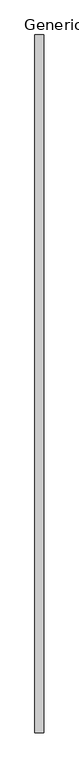
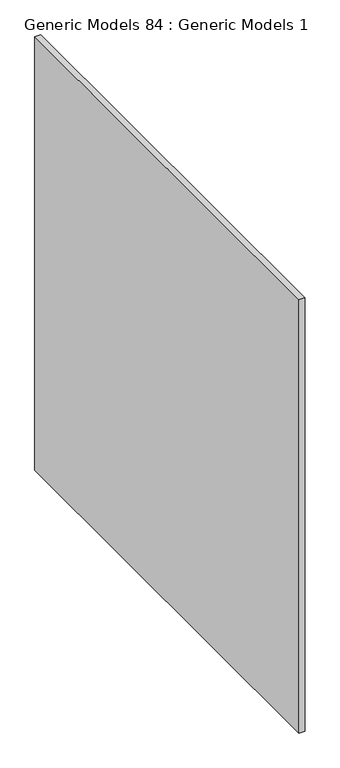
"""IFC4 building model written with IfcOpenShell, lengths in millimetres: proxy geometry, Generic Models 84 : Generic Models 1."""

from ifc_helpers import new_model, si_unit, frame, origin, place, context, project, spatial, polyline, outline, extrude, source, transform, mapped, element, save


def generic_models_84_generic_models_1_80fe95b7(model_context):
    return source(origin(), model_context, "Body", "SweptSolid", [
        extrude(outline(polyline([(48432.6703765, 0.0), (48416.7953765, 0.0), (48416.7953765, 1219.2), (48432.6703765, 1219.2), (48432.6703765, 0.0)])), frame((0.0, 0.0, 34.479891), z_axis=(0.0, 0.0, 1.0), x_axis=(1.0, 0.0, 0.0)), (0.0, 0.0, 1.0), 1219.2),
    ])


if __name__ == "__main__":
    model = new_model("IFC4")
    model_context = context("Model", 3, world=origin())
    ifc_project = project(units=[si_unit("LENGTHUNIT", "METRE", prefix="MILLI")], contexts=[model_context])
    site = spatial("IfcSite", under=ifc_project)
    building = spatial("IfcBuilding", under=site)
    placement = place(None, origin())
    generic_models_84_generic_models_1_shape = generic_models_84_generic_models_1_80fe95b7(model_context)
    element("IfcBuildingElementProxy", 1, Name="Generic Models 84 : Generic Models 1", ObjectType="Generic Models 84 : Generic Models 1", at=placement, inside=building, context=model_context, shape_type="MappedRepresentation", body=[
        mapped(generic_models_84_generic_models_1_shape, transform((0.0, 0.0, 0.0), x_axis=(1.0, 0.0, 0.0), y_axis=(0.0, 1.0, 0.0), z_axis=(0.0, 0.0, 1.0))),
    ])
    save(model, "model.ifc")

# Revit data of these elements
# Element 1 (IfcBuildingElementProxy, "Generic Models 84 : Generic Models 1")
#   Materials on its faces: "5/8\" GYP. BD"
# Materials
#   "5/8\" GYP. BD": class "Generic", colour RGB 136 135 132, transparency 0, Description = "Gypsum Wall Board", Cost = 0
